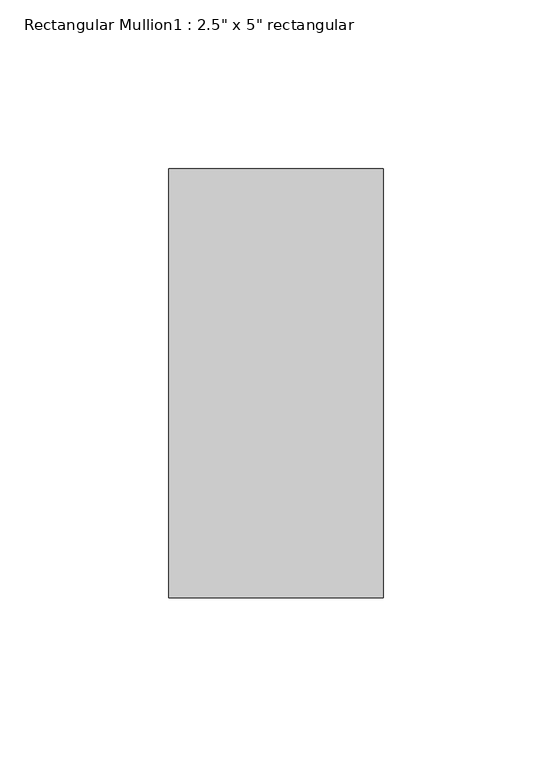
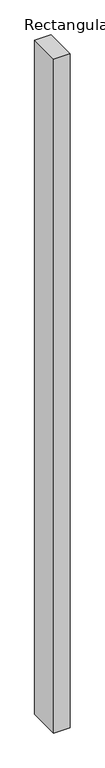
"""IFC4 building model written with IfcOpenShell, lengths in millimetres: member geometry."""

from ifc_helpers import new_model, si_unit, frame, origin, place, context, project, spatial, polyline, outline, extrude, source, transform, mapped, element, save


def member_923d5781(model_context):
    return source(origin(), model_context, "Body", "SweptSolid", [
        extrude(outline(polyline([(31.75, 63.5), (31.75, -63.5), (-31.75, -63.5), (-31.75, 63.5), (31.75, 63.5)])), frame((0.0, 0.0, -2743.2), z_axis=(0.0, 0.0, 1.0), x_axis=(1.0, 0.0, 0.0)), (0.0, 0.0, 1.0), 2743.2),
    ])


if __name__ == "__main__":
    model = new_model("IFC4")
    model_context = context("Model", 3, world=origin())
    ifc_project = project(units=[si_unit("LENGTHUNIT", "METRE", prefix="MILLI")], contexts=[model_context])
    site = spatial("IfcSite", under=ifc_project)
    building = spatial("IfcBuilding", under=site)
    placement = place(None, origin())
    member_shape = member_923d5781(model_context)
    element("IfcMember", 1, ObjectType="Rectangular Mullion1 : 2.5\" x 5\" rectangular", at=placement, inside=building, context=model_context, shape_type="MappedRepresentation", body=[
        mapped(member_shape, transform((0.0, 0.0, 0.0), x_axis=(1.0, 0.0, 0.0), y_axis=(0.0, 1.0, 0.0), z_axis=(0.0, 0.0, 1.0))),
    ])
    save(model, "model.ifc")

# Revit data of these elements
# Type "Rectangular Mullion1 : 2.5\" x 5\" rectangular"
#   built-in parameter 1007304 = 0.416667 (stored number, unit not read)
#   built-in parameter 1007301 = 0.104167 (stored number, unit not read)
#   built-in parameter 1007300 = 0.104167 (stored number, unit not read)
# Element 1 (IfcMember, "Rectangular Mullion1 : 2.5\" x 5\" rectangular")
#   Materials on its faces: "support-frame"
# Materials
#   "support-frame": class "Unassigned", colour RGB 233 233 233, transparency 0, Cost = 0
